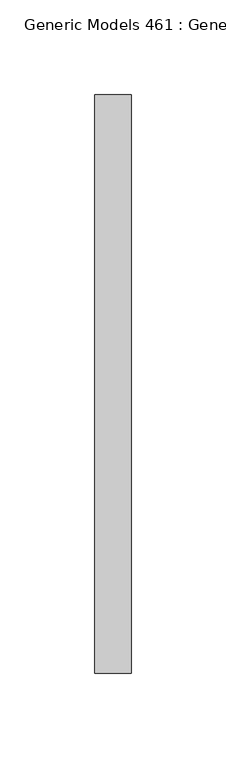
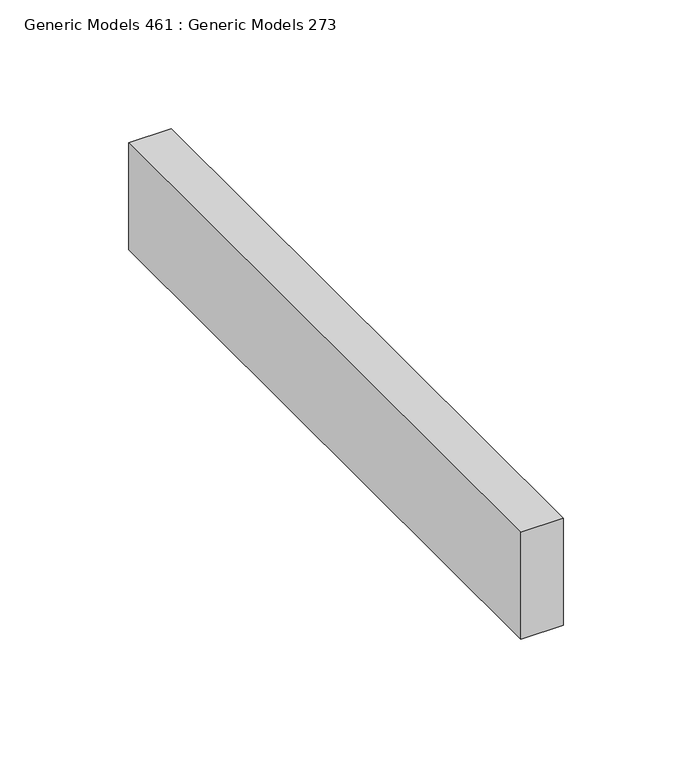
"""IFC4 building model written with IfcOpenShell, lengths in millimetres: proxy geometry, Generic Models 461 : Generic Models 273."""

from ifc_helpers import new_model, si_unit, frame, origin, place, context, project, spatial, polyline, outline, extrude, source, transform, mapped, element, save


def generic_models_461_generic_models_273_a027c428(model_context):
    return source(origin(), model_context, "Body", "SweptSolid", [
        extrude(outline(polyline([(1642.0931224, 4564.8872686), (1661.1431224, 4564.8872686), (1661.1431224, 4260.0872686), (1642.0931224, 4260.0872686), (1642.0931224, 4564.8872686)])), frame((0.0, 0.0, 123432.2376949), z_axis=(0.0, 0.0, 1.0), x_axis=(1.0, 0.0, 0.0)), (0.0, 0.0, 1.0), 50.8932516),
    ])


if __name__ == "__main__":
    model = new_model("IFC4")
    model_context = context("Model", 3, world=origin())
    ifc_project = project(units=[si_unit("LENGTHUNIT", "METRE", prefix="MILLI")], contexts=[model_context])
    site = spatial("IfcSite", under=ifc_project)
    building = spatial("IfcBuilding", under=site)
    placement = place(None, origin())
    generic_models_461_generic_models_273_shape = generic_models_461_generic_models_273_a027c428(model_context)
    element("IfcBuildingElementProxy", 1, Name="Generic Models 461 : Generic Models 273", ObjectType="Generic Models 461 : Generic Models 273", at=placement, inside=building, context=model_context, shape_type="MappedRepresentation", body=[
        mapped(generic_models_461_generic_models_273_shape, transform((0.0, 0.0, 0.0), x_axis=(1.0, 0.0, 0.0), y_axis=(0.0, 1.0, 0.0), z_axis=(0.0, 0.0, 1.0))),
    ])
    save(model, "model.ifc")

# Revit data of these elements
# Element 1 (IfcBuildingElementProxy, "Generic Models 461 : Generic Models 273")
#   Materials on its faces: "_TREATED BLOCKING AS REQUIRED"
# Materials
#   "_TREATED BLOCKING AS REQUIRED": class "Generic", colour RGB 177 130 114, transparency 0, Cost = 0
